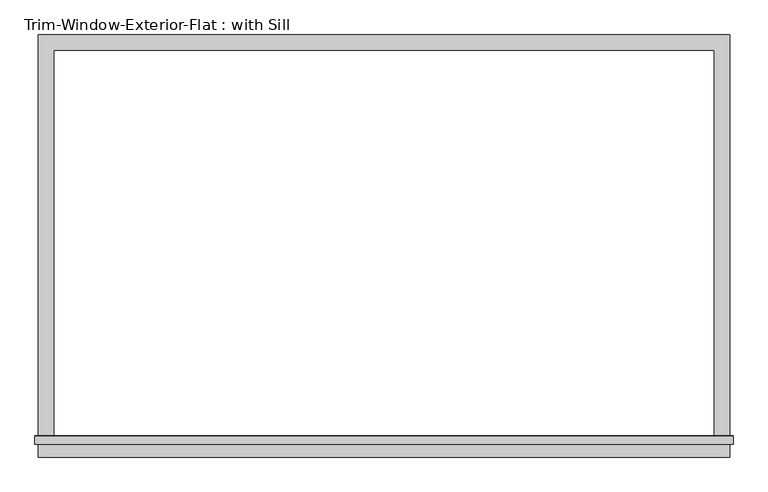
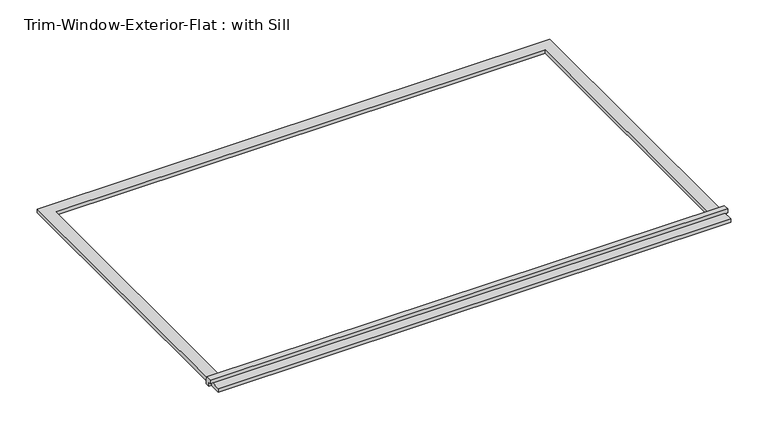
"""IFC4 building model written with IfcOpenShell, lengths in millimetres: proxy geometry, Trim-Window-Exterior-Flat : with Sill."""

import ifcopenshell
import ifcopenshell.guid

model = None  # the IFC model being written
_history = None  # IfcOwnerHistory: only IFC2X3 demands one
_inside = {}  # id of a spatial element -> (the spatial element, [elements in it])
_under = {}  # id of a project, library or spatial element -> (it, [spatial elements below it])
_declared = {}  # id of a project -> (the project, [libraries it declares])
_typed = {}  # id of a type object -> (the type object, [elements of that type])
_made_of = {}  # id of a material, layer set ... -> (it, [elements and type objects made of it])


def new_model(schema):
    """Start an empty IFC model of exactly this schema.

    Asked for "IFC4X3", IfcOpenShell would pick the latest addendum, in which some entities
    have other attributes; the version numbers below select the first issue.
    IFC2X3 requires an IfcOwnerHistory on every rooted entity: one is made here for all.
    """
    global model, _history
    if schema == "IFC4X3":
        model = ifcopenshell.file(schema_version=(4, 3, 0, 0))
    else:
        model = ifcopenshell.file(schema=schema)
    _inside.clear()
    _under.clear()
    _declared.clear()
    _typed.clear()
    _made_of.clear()
    _history = None
    if model.schema == "IFC2X3":
        org = make("IfcOrganization", Name="unknown")
        user = make(
            "IfcPersonAndOrganization",
            ThePerson=make("IfcPerson", FamilyName="unknown"),
            TheOrganization=org,
        )
        app = make(
            "IfcApplication",
            ApplicationDeveloper=org,
            Version="unknown",
            ApplicationFullName="unknown",
            ApplicationIdentifier="unknown",
        )
        _history = make(
            "IfcOwnerHistory",
            OwningUser=user,
            OwningApplication=app,
            ChangeAction="ADDED",
            CreationDate=0,
        )
    return model


def make(cls, **values):
    """One entity of the class cls with the attributes given. An attribute that is None is left unset."""
    return model.create_entity(
        cls, **{name: value for name, value in values.items() if value is not None}
    )


def rooted(cls, **values):
    """An entity with a GlobalId (a new one), such as an element, a storey or a relation."""
    return make(cls, GlobalId=ifcopenshell.guid.new(), OwnerHistory=_history, **values)


def si_unit(unit_type, name, prefix=None):
    """IfcSIUnit, for example si_unit("LENGTHUNIT", "METRE", prefix="MILLI")."""
    return make("IfcSIUnit", UnitType=unit_type, Prefix=prefix, Name=name)


def assignment(units):
    """IfcUnitAssignment: the units of a project."""
    return None if units is None else make("IfcUnitAssignment", Units=units)


def point(xyz):
    """IfcCartesianPoint."""
    return None if xyz is None else make("IfcCartesianPoint", Coordinates=xyz)


def direction(xyz):
    """IfcDirection."""
    return None if xyz is None else make("IfcDirection", DirectionRatios=xyz)


def frame(location, z_axis=None, x_axis=None):
    """IfcAxis2Placement3D, a coordinate frame: its origin and axes. An axis left out is left unset."""
    return make(
        "IfcAxis2Placement3D",
        Location=point(location),
        Axis=direction(z_axis),
        RefDirection=direction(x_axis),
    )


def origin():
    """The frame at (0, 0, 0) with its axes left unset."""
    return frame((0.0, 0.0, 0.0))


def origin_with_axes():
    """The frame at (0, 0, 0) with the z axis (0, 0, 1) and the x axis (1, 0, 0) written out."""
    return frame((0.0, 0.0, 0.0), z_axis=(0.0, 0.0, 1.0), x_axis=(1.0, 0.0, 0.0))


def place(relative_to, where):
    """IfcLocalPlacement: puts the frame where relative to a parent placement (None: the world)."""
    return make(
        "IfcLocalPlacement", PlacementRelTo=relative_to, RelativePlacement=where
    )


def context(
    kind, dimensions, precision=None, world=None, true_north=None, identifier=None
):
    """IfcGeometricRepresentationContext, for example the 3D "Model" context."""
    return make(
        "IfcGeometricRepresentationContext",
        ContextIdentifier=identifier,
        ContextType=kind,
        CoordinateSpaceDimension=dimensions,
        Precision=precision,
        WorldCoordinateSystem=world,
        TrueNorth=true_north,
    )


def project(units=None, contexts=None):
    """IfcProject with its units and contexts."""
    return rooted(
        "IfcProject",
        Name="project",
        RepresentationContexts=contexts,
        UnitsInContext=assignment(units),
    )


def spatial(cls, under=None, at=None, **own):
    """A site, building, storey or space (cls), placed at a placement, below another one or the project."""
    s = rooted(cls, ObjectPlacement=at, **own)
    if under is not None:
        _under.setdefault(under.id(), (under, []))[1].append(s)
    return s


def polyline(points):
    """IfcPolyline through the points."""
    return make("IfcPolyline", Points=[point(p) for p in points])


def outline(outer, holes=None, kind="AREA"):
    """IfcArbitraryClosedProfileDef: a profile drawn as a closed curve; with holes, ...WithVoids."""
    if holes is None:
        return make("IfcArbitraryClosedProfileDef", ProfileType=kind, OuterCurve=outer)
    return make(
        "IfcArbitraryProfileDefWithVoids",
        ProfileType=kind,
        OuterCurve=outer,
        InnerCurves=holes,
    )


def extrude(swept, where, along, depth):
    """IfcExtrudedAreaSolid: the profile swept, set in the frame where, extruded along a direction by depth."""
    return make(
        "IfcExtrudedAreaSolid",
        SweptArea=swept,
        Position=where,
        ExtrudedDirection=direction(along),
        Depth=depth,
    )


def shape(context_of_items, identifier, shape_type, items):
    """IfcShapeRepresentation: the items that make up one representation, for example the "Body"."""
    return make(
        "IfcShapeRepresentation",
        ContextOfItems=context_of_items,
        RepresentationIdentifier=identifier,
        RepresentationType=shape_type,
        Items=items,
    )


def source(mapping_origin, context_of_items, identifier, shape_type, items):
    """IfcRepresentationMap: a shape defined once, which mapped items show again and again."""
    return make(
        "IfcRepresentationMap",
        MappingOrigin=mapping_origin,
        MappedRepresentation=shape(context_of_items, identifier, shape_type, items),
    )


def transform(
    local_origin,
    x_axis=None,
    y_axis=None,
    z_axis=None,
    scale=None,
    scale2=None,
    scale3=None,
    uniform=True,
):
    """IfcCartesianTransformationOperator3D, or its non-uniform kind. x_axis, y_axis, z_axis: its Axis1, 2, 3."""
    if uniform:
        return make(
            "IfcCartesianTransformationOperator3D",
            Axis1=direction(x_axis),
            Axis2=direction(y_axis),
            LocalOrigin=point(local_origin),
            Scale=scale,
            Axis3=direction(z_axis),
        )
    return make(
        "IfcCartesianTransformationOperator3DnonUniform",
        Axis1=direction(x_axis),
        Axis2=direction(y_axis),
        LocalOrigin=point(local_origin),
        Scale=scale,
        Axis3=direction(z_axis),
        Scale2=scale2,
        Scale3=scale3,
    )


def mapped(mapping_source, mapping_target):
    """IfcMappedItem: shows the shape of a source again, moved by a transform."""
    return make(
        "IfcMappedItem", MappingSource=mapping_source, MappingTarget=mapping_target
    )


def made_of(thing, what):
    """Note that an element or type object is made of a material, layer set ...; save() writes the relation."""
    if what is not None:
        _made_of.setdefault(what.id(), (what, []))[1].append(thing)
    return thing


def element(
    cls,
    number,
    at=None,
    inside=None,
    cuts=None,
    type_object=None,
    material=None,
    context=None,
    identifier="Body",
    shape_type=None,
    held_by="IfcProductDefinitionShape",
    body=None,
    shapes=None,
    **own,
):
    """One element of the class cls, such as IfcWall. Its Tag is "e" and its number.

    at: its placement. inside: the storey or other place that contains it. cuts: it is an
    opening in that element (IfcRelVoidsElement). A single representation is given by context,
    identifier, shape_type and body (its items); several are given by shapes. held_by: the class
    of the entity that holds the representations. save() writes the other relations.
    """
    e = rooted(cls, Tag="e%d" % number, ObjectPlacement=at, **own)
    if body is not None:
        shapes = [shape(context, identifier, shape_type, body)]
    if shapes is not None:
        e.Representation = make(held_by, Representations=shapes)
    if inside is not None:
        _inside.setdefault(inside.id(), (inside, []))[1].append(e)
    if cuts is not None:
        rooted(
            "IfcRelVoidsElement", RelatingBuildingElement=cuts, RelatedOpeningElement=e
        )
    if type_object is not None:
        _typed.setdefault(type_object.id(), (type_object, []))[1].append(e)
    return made_of(e, material)


def aggregate(whole, parts):
    """IfcRelAggregates: a whole, such as a stair, and the parts it consists of."""
    return rooted("IfcRelAggregates", RelatingObject=whole, RelatedObjects=parts)


def save(model, path):
    """Write the relations noted so far, then the file.

    IfcRelAggregates (storeys below a building ...), IfcRelContainedInSpatialStructure (elements
    in a storey), IfcRelDefinesByType, IfcRelAssociatesMaterial and IfcRelDeclares: one each for
    every whole, place, type object, material and project.
    """
    for whole, parts in _under.values():
        aggregate(whole, parts)
    for where, things in _inside.values():
        rooted(
            "IfcRelContainedInSpatialStructure",
            RelatedElements=things,
            RelatingStructure=where,
        )
    for kind, things in _typed.values():
        rooted("IfcRelDefinesByType", RelatedObjects=things, RelatingType=kind)
    for what, things in _made_of.values():
        rooted("IfcRelAssociatesMaterial", RelatedObjects=things, RelatingMaterial=what)
    for by, libraries in _declared.values():
        rooted("IfcRelDeclares", RelatingContext=by, RelatedDefinitions=libraries)
    model.write(path)


def trim_window_exterior_flat_with_sill_cc36b48f(model_context):
    return source(origin(), model_context, "Body", "SweptSolid", [
        extrude(outline(polyline([(1276.35, -1444.5823709), (1276.35, -1501.7323709), (-1276.35, -1501.7323709), (-1276.35, -1444.5823709), (1276.35, -1444.5823709)])), origin_with_axes(), (0.0, 0.0, 1.0), 19.05),
        extrude(outline(polyline([(-1454.15, 38.1), (-1424.8580645, 38.1), (-1422.4, 19.05), (-1422.4, 0.0), (-1444.5823709, 0.0), (-1444.5823709, 19.05), (-1454.15, 19.05), (-1454.15, 38.1)])), frame((-1289.05, 0.0, 0.0), z_axis=(1.0, 0.0, 0.0), x_axis=(0.0, 1.0, 0.0)), (0.0, 0.0, 1.0), 2578.1),
        extrude(outline(polyline([(-1276.35, 57.15), (1276.35, 57.15), (1276.35, -1422.4), (1219.2, -1422.4), (1219.2, 0.0), (-1219.2, 0.0), (-1219.2, -1422.4), (-1276.35, -1422.4), (-1276.35, 57.15)])), origin_with_axes(), (0.0, 0.0, 1.0), 19.05),
    ])


if __name__ == "__main__":
    model = new_model("IFC4")
    model_context = context("Model", 3, world=origin())
    ifc_project = project(units=[si_unit("LENGTHUNIT", "METRE", prefix="MILLI")], contexts=[model_context])
    site = spatial("IfcSite", under=ifc_project)
    building = spatial("IfcBuilding", under=site)
    placement = place(None, origin())
    trim_window_exterior_flat_with_sill_shape = trim_window_exterior_flat_with_sill_cc36b48f(model_context)
    element("IfcBuildingElementProxy", 1, Name="Trim-Window-Exterior-Flat : with Sill", ObjectType="Trim-Window-Exterior-Flat : with Sill", at=placement, inside=building, context=model_context, shape_type="MappedRepresentation", body=[
        mapped(trim_window_exterior_flat_with_sill_shape, transform((0.0, 0.0, 0.0), x_axis=(1.0, 0.0, 0.0), y_axis=(0.0, 1.0, 0.0), z_axis=(0.0, 0.0, 1.0))),
    ])
    save(model, "model.ifc")

# Revit data of these elements
# Type "Trim-Window-Exterior-Flat : with Sill"
#   Trim Width = 0' - 2 1/4"
#   Trim Thickness_Picture Frame = 0' - 1 1/4"
#   Trim Thickness_with Sill = 0' - 0 3/4"
#   Sill Thickness = 0' - 1 1/4"
#   Opening Width [instance default] = 2' - 0"
#   Opening Height [instance default] = 3' - 0"
#   Default Elevation = 4' - 0"
#   Sill = yes
#   Picture Frame = no
#   Trim Material [instance default] = none
# Element 1 (IfcBuildingElementProxy, "Trim-Window-Exterior-Flat : with Sill")
#   Opening Width = 8' - 0"
#   Opening Height = 4' - 8"
#   Trim Material = Clad - White
#   Materials on its faces: "Clad - White"
# Materials
#   "Clad - White": class "Wood", colour RGB 242 242 238, transparency 0, Cost = 0
